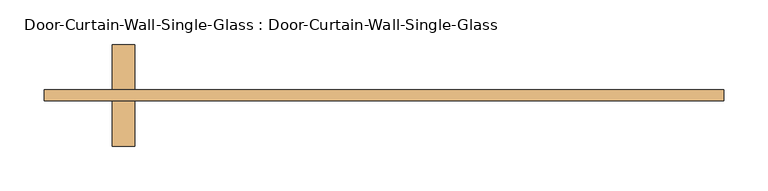
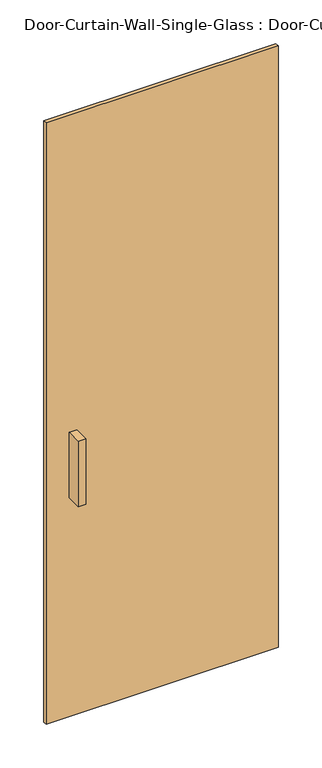
"""IFC4 building model written with IfcOpenShell, lengths in millimetres: door geometry, Door-Curtain-Wall-Single-Glass : Door-Curtain-Wall-Single-Glass."""

import ifcopenshell
import ifcopenshell.guid

model = None  # the IFC model being written
_history = None  # IfcOwnerHistory: only IFC2X3 demands one
_inside = {}  # id of a spatial element -> (the spatial element, [elements in it])
_under = {}  # id of a project, library or spatial element -> (it, [spatial elements below it])
_declared = {}  # id of a project -> (the project, [libraries it declares])
_typed = {}  # id of a type object -> (the type object, [elements of that type])
_made_of = {}  # id of a material, layer set ... -> (it, [elements and type objects made of it])


def new_model(schema):
    """Start an empty IFC model of exactly this schema.

    Asked for "IFC4X3", IfcOpenShell would pick the latest addendum, in which some entities
    have other attributes; the version numbers below select the first issue.
    IFC2X3 requires an IfcOwnerHistory on every rooted entity: one is made here for all.
    """
    global model, _history
    if schema == "IFC4X3":
        model = ifcopenshell.file(schema_version=(4, 3, 0, 0))
    else:
        model = ifcopenshell.file(schema=schema)
    _inside.clear()
    _under.clear()
    _declared.clear()
    _typed.clear()
    _made_of.clear()
    _history = None
    if model.schema == "IFC2X3":
        org = make("IfcOrganization", Name="unknown")
        user = make(
            "IfcPersonAndOrganization",
            ThePerson=make("IfcPerson", FamilyName="unknown"),
            TheOrganization=org,
        )
        app = make(
            "IfcApplication",
            ApplicationDeveloper=org,
            Version="unknown",
            ApplicationFullName="unknown",
            ApplicationIdentifier="unknown",
        )
        _history = make(
            "IfcOwnerHistory",
            OwningUser=user,
            OwningApplication=app,
            ChangeAction="ADDED",
            CreationDate=0,
        )
    return model


def make(cls, **values):
    """One entity of the class cls with the attributes given. An attribute that is None is left unset."""
    return model.create_entity(
        cls, **{name: value for name, value in values.items() if value is not None}
    )


def rooted(cls, **values):
    """An entity with a GlobalId (a new one), such as an element, a storey or a relation."""
    return make(cls, GlobalId=ifcopenshell.guid.new(), OwnerHistory=_history, **values)


def si_unit(unit_type, name, prefix=None):
    """IfcSIUnit, for example si_unit("LENGTHUNIT", "METRE", prefix="MILLI")."""
    return make("IfcSIUnit", UnitType=unit_type, Prefix=prefix, Name=name)


def assignment(units):
    """IfcUnitAssignment: the units of a project."""
    return None if units is None else make("IfcUnitAssignment", Units=units)


def point(xyz):
    """IfcCartesianPoint."""
    return None if xyz is None else make("IfcCartesianPoint", Coordinates=xyz)


def direction(xyz):
    """IfcDirection."""
    return None if xyz is None else make("IfcDirection", DirectionRatios=xyz)


def frame(location, z_axis=None, x_axis=None):
    """IfcAxis2Placement3D, a coordinate frame: its origin and axes. An axis left out is left unset."""
    return make(
        "IfcAxis2Placement3D",
        Location=point(location),
        Axis=direction(z_axis),
        RefDirection=direction(x_axis),
    )


def origin():
    """The frame at (0, 0, 0) with its axes left unset."""
    return frame((0.0, 0.0, 0.0))


def origin_with_axes():
    """The frame at (0, 0, 0) with the z axis (0, 0, 1) and the x axis (1, 0, 0) written out."""
    return frame((0.0, 0.0, 0.0), z_axis=(0.0, 0.0, 1.0), x_axis=(1.0, 0.0, 0.0))


def place(relative_to, where):
    """IfcLocalPlacement: puts the frame where relative to a parent placement (None: the world)."""
    return make(
        "IfcLocalPlacement", PlacementRelTo=relative_to, RelativePlacement=where
    )


def context(
    kind, dimensions, precision=None, world=None, true_north=None, identifier=None
):
    """IfcGeometricRepresentationContext, for example the 3D "Model" context."""
    return make(
        "IfcGeometricRepresentationContext",
        ContextIdentifier=identifier,
        ContextType=kind,
        CoordinateSpaceDimension=dimensions,
        Precision=precision,
        WorldCoordinateSystem=world,
        TrueNorth=true_north,
    )


def project(units=None, contexts=None):
    """IfcProject with its units and contexts."""
    return rooted(
        "IfcProject",
        Name="project",
        RepresentationContexts=contexts,
        UnitsInContext=assignment(units),
    )


def spatial(cls, under=None, at=None, **own):
    """A site, building, storey or space (cls), placed at a placement, below another one or the project."""
    s = rooted(cls, ObjectPlacement=at, **own)
    if under is not None:
        _under.setdefault(under.id(), (under, []))[1].append(s)
    return s


def polyline(points):
    """IfcPolyline through the points."""
    return make("IfcPolyline", Points=[point(p) for p in points])


def outline(outer, holes=None, kind="AREA"):
    """IfcArbitraryClosedProfileDef: a profile drawn as a closed curve; with holes, ...WithVoids."""
    if holes is None:
        return make("IfcArbitraryClosedProfileDef", ProfileType=kind, OuterCurve=outer)
    return make(
        "IfcArbitraryProfileDefWithVoids",
        ProfileType=kind,
        OuterCurve=outer,
        InnerCurves=holes,
    )


def extrude(swept, where, along, depth):
    """IfcExtrudedAreaSolid: the profile swept, set in the frame where, extruded along a direction by depth."""
    return make(
        "IfcExtrudedAreaSolid",
        SweptArea=swept,
        Position=where,
        ExtrudedDirection=direction(along),
        Depth=depth,
    )


def shape(context_of_items, identifier, shape_type, items):
    """IfcShapeRepresentation: the items that make up one representation, for example the "Body"."""
    return make(
        "IfcShapeRepresentation",
        ContextOfItems=context_of_items,
        RepresentationIdentifier=identifier,
        RepresentationType=shape_type,
        Items=items,
    )


def source(mapping_origin, context_of_items, identifier, shape_type, items):
    """IfcRepresentationMap: a shape defined once, which mapped items show again and again."""
    return make(
        "IfcRepresentationMap",
        MappingOrigin=mapping_origin,
        MappedRepresentation=shape(context_of_items, identifier, shape_type, items),
    )


def transform(
    local_origin,
    x_axis=None,
    y_axis=None,
    z_axis=None,
    scale=None,
    scale2=None,
    scale3=None,
    uniform=True,
):
    """IfcCartesianTransformationOperator3D, or its non-uniform kind. x_axis, y_axis, z_axis: its Axis1, 2, 3."""
    if uniform:
        return make(
            "IfcCartesianTransformationOperator3D",
            Axis1=direction(x_axis),
            Axis2=direction(y_axis),
            LocalOrigin=point(local_origin),
            Scale=scale,
            Axis3=direction(z_axis),
        )
    return make(
        "IfcCartesianTransformationOperator3DnonUniform",
        Axis1=direction(x_axis),
        Axis2=direction(y_axis),
        LocalOrigin=point(local_origin),
        Scale=scale,
        Axis3=direction(z_axis),
        Scale2=scale2,
        Scale3=scale3,
    )


def mapped(mapping_source, mapping_target):
    """IfcMappedItem: shows the shape of a source again, moved by a transform."""
    return make(
        "IfcMappedItem", MappingSource=mapping_source, MappingTarget=mapping_target
    )


def made_of(thing, what):
    """Note that an element or type object is made of a material, layer set ...; save() writes the relation."""
    if what is not None:
        _made_of.setdefault(what.id(), (what, []))[1].append(thing)
    return thing


def element(
    cls,
    number,
    at=None,
    inside=None,
    cuts=None,
    type_object=None,
    material=None,
    context=None,
    identifier="Body",
    shape_type=None,
    held_by="IfcProductDefinitionShape",
    body=None,
    shapes=None,
    **own,
):
    """One element of the class cls, such as IfcWall. Its Tag is "e" and its number.

    at: its placement. inside: the storey or other place that contains it. cuts: it is an
    opening in that element (IfcRelVoidsElement). A single representation is given by context,
    identifier, shape_type and body (its items); several are given by shapes. held_by: the class
    of the entity that holds the representations. save() writes the other relations.
    """
    e = rooted(cls, Tag="e%d" % number, ObjectPlacement=at, **own)
    if body is not None:
        shapes = [shape(context, identifier, shape_type, body)]
    if shapes is not None:
        e.Representation = make(held_by, Representations=shapes)
    if inside is not None:
        _inside.setdefault(inside.id(), (inside, []))[1].append(e)
    if cuts is not None:
        rooted(
            "IfcRelVoidsElement", RelatingBuildingElement=cuts, RelatedOpeningElement=e
        )
    if type_object is not None:
        _typed.setdefault(type_object.id(), (type_object, []))[1].append(e)
    return made_of(e, material)


def aggregate(whole, parts):
    """IfcRelAggregates: a whole, such as a stair, and the parts it consists of."""
    return rooted("IfcRelAggregates", RelatingObject=whole, RelatedObjects=parts)


def save(model, path):
    """Write the relations noted so far, then the file.

    IfcRelAggregates (storeys below a building ...), IfcRelContainedInSpatialStructure (elements
    in a storey), IfcRelDefinesByType, IfcRelAssociatesMaterial and IfcRelDeclares: one each for
    every whole, place, type object, material and project.
    """
    for whole, parts in _under.values():
        aggregate(whole, parts)
    for where, things in _inside.values():
        rooted(
            "IfcRelContainedInSpatialStructure",
            RelatedElements=things,
            RelatingStructure=where,
        )
    for kind, things in _typed.values():
        rooted("IfcRelDefinesByType", RelatedObjects=things, RelatingType=kind)
    for what, things in _made_of.values():
        rooted("IfcRelAssociatesMaterial", RelatedObjects=things, RelatingMaterial=what)
    for by, libraries in _declared.values():
        rooted("IfcRelDeclares", RelatingContext=by, RelatedDefinitions=libraries)
    model.write(path)


def door_curtain_wall_single_glass_door_curtain_wall_single_e3b46ede(model_context):
    return source(origin(), model_context, "Body", "SweptSolid", [
        extrude(outline(polyline([(382.3136177, 0.0), (-382.3136177, 0.0), (-382.3136177, 12.7), (382.3136177, 12.7), (382.3136177, 0.0)])), origin_with_axes(), (0.0, 0.0, 1.0), 2095.5),
        extrude(outline(polyline([(-280.7136177, 63.5), (-280.7136177, 12.7), (-306.1136177, 12.7), (-306.1136177, 63.5), (-280.7136177, 63.5)])), frame((0.0, 0.0, 762.0), z_axis=(0.0, 0.0, 1.0), x_axis=(1.0, 0.0, 0.0)), (0.0, 0.0, 1.0), 228.6),
        extrude(outline(polyline([(-306.1136177, -50.8), (-306.1136177, 0.0), (-280.7136177, 0.0), (-280.7136177, -50.8), (-306.1136177, -50.8)])), frame((0.0, 0.0, 762.0), z_axis=(0.0, 0.0, 1.0), x_axis=(1.0, 0.0, 0.0)), (0.0, 0.0, 1.0), 228.6),
    ])


if __name__ == "__main__":
    model = new_model("IFC4")
    model_context = context("Model", 3, world=origin())
    ifc_project = project(units=[si_unit("LENGTHUNIT", "METRE", prefix="MILLI")], contexts=[model_context])
    site = spatial("IfcSite", under=ifc_project)
    building = spatial("IfcBuilding", under=site)
    placement = place(None, origin())
    door_curtain_wall_single_glass_door_curtain_wall_single_shape = door_curtain_wall_single_glass_door_curtain_wall_single_e3b46ede(model_context)
    element("IfcDoor", 1, ObjectType="Door-Curtain-Wall-Single-Glass : Door-Curtain-Wall-Single-Glass", at=placement, inside=building, context=model_context, shape_type="MappedRepresentation", body=[
        mapped(door_curtain_wall_single_glass_door_curtain_wall_single_shape, transform((0.0, 0.0, 0.0), x_axis=(1.0, 0.0, 0.0), y_axis=(0.0, 1.0, 0.0), z_axis=(0.0, 0.0, 1.0))),
    ])
    save(model, "model.ifc")

# Revit data of these elements
# Type "Door-Curtain-Wall-Single-Glass : Door-Curtain-Wall-Single-Glass"
#   Type Mark = "9"
#   Assembly Code = "B2030100"
#   Analytic Construction = "<None>"
#   Width [instance default] = 3' - 0"
#   Thermal Resistance (R) = 10.0000 (h·ft²·°F)/BTU
#   Swing Angle [instance default] = 90.00°
#   Heat Transfer Coefficient (U) = 0.1000 BTU/(h·ft²·°F)
#   Offset = 0' - 0"
#   Define Thermal Properties by = 1
#   Function = 1
#   Door Handle Material = Aluminum
#   Glazing = Glass
#   Visual Light Transmittance = 0
#   Solar Heat Gain Coefficient = 0
#   Construction Type Id = ""
# Element 1 (IfcDoor, "Door-Curtain-Wall-Single-Glass : Door-Curtain-Wall-Single-Glass")
#   Width = 2' - 6.10343"
#   Materials on its faces: "Aluminum", "Glass"
# Materials
#   "Aluminum": class "Metal", colour RGB 247 247 247, transparency 0, Description = "Aluminum 6061", Cost = 0
#   "Glass": class "Glass", colour RGB 0 128 192, transparency 0.75, Description = "Soda Lime Glass", Cost = 0
